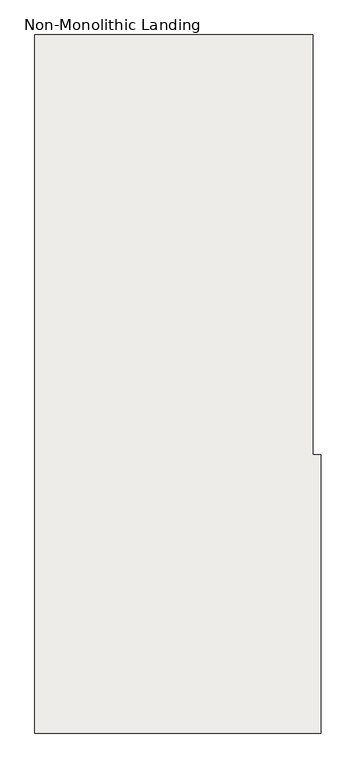
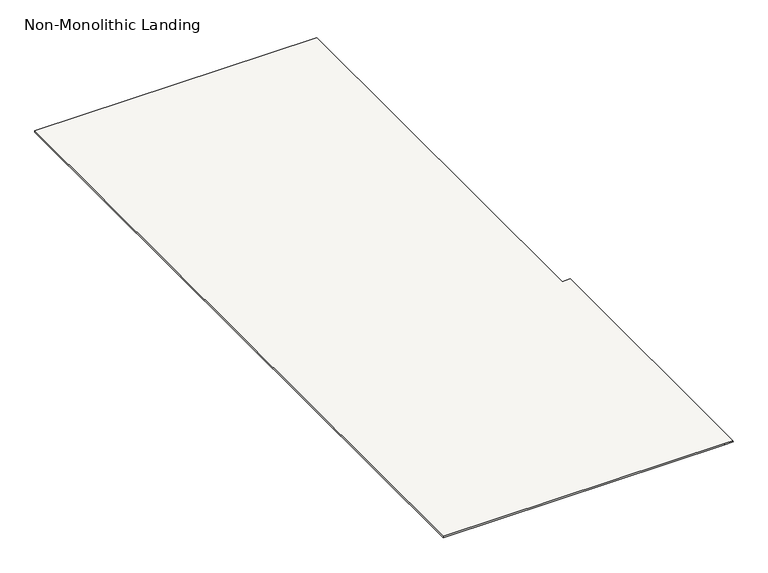
"""IFC4 building model written with IfcOpenShell, lengths in millimetres: slab geometry, Non-Monolithic Landing."""

import ifcopenshell
import ifcopenshell.guid

model = None  # the IFC model being written
_history = None  # IfcOwnerHistory: only IFC2X3 demands one
_inside = {}  # id of a spatial element -> (the spatial element, [elements in it])
_under = {}  # id of a project, library or spatial element -> (it, [spatial elements below it])
_declared = {}  # id of a project -> (the project, [libraries it declares])
_typed = {}  # id of a type object -> (the type object, [elements of that type])
_made_of = {}  # id of a material, layer set ... -> (it, [elements and type objects made of it])


def new_model(schema):
    """Start an empty IFC model of exactly this schema.

    Asked for "IFC4X3", IfcOpenShell would pick the latest addendum, in which some entities
    have other attributes; the version numbers below select the first issue.
    IFC2X3 requires an IfcOwnerHistory on every rooted entity: one is made here for all.
    """
    global model, _history
    if schema == "IFC4X3":
        model = ifcopenshell.file(schema_version=(4, 3, 0, 0))
    else:
        model = ifcopenshell.file(schema=schema)
    _inside.clear()
    _under.clear()
    _declared.clear()
    _typed.clear()
    _made_of.clear()
    _history = None
    if model.schema == "IFC2X3":
        org = make("IfcOrganization", Name="unknown")
        user = make(
            "IfcPersonAndOrganization",
            ThePerson=make("IfcPerson", FamilyName="unknown"),
            TheOrganization=org,
        )
        app = make(
            "IfcApplication",
            ApplicationDeveloper=org,
            Version="unknown",
            ApplicationFullName="unknown",
            ApplicationIdentifier="unknown",
        )
        _history = make(
            "IfcOwnerHistory",
            OwningUser=user,
            OwningApplication=app,
            ChangeAction="ADDED",
            CreationDate=0,
        )
    return model


def make(cls, **values):
    """One entity of the class cls with the attributes given. An attribute that is None is left unset."""
    return model.create_entity(
        cls, **{name: value for name, value in values.items() if value is not None}
    )


def rooted(cls, **values):
    """An entity with a GlobalId (a new one), such as an element, a storey or a relation."""
    return make(cls, GlobalId=ifcopenshell.guid.new(), OwnerHistory=_history, **values)


def si_unit(unit_type, name, prefix=None):
    """IfcSIUnit, for example si_unit("LENGTHUNIT", "METRE", prefix="MILLI")."""
    return make("IfcSIUnit", UnitType=unit_type, Prefix=prefix, Name=name)


def assignment(units):
    """IfcUnitAssignment: the units of a project."""
    return None if units is None else make("IfcUnitAssignment", Units=units)


def point(xyz):
    """IfcCartesianPoint."""
    return None if xyz is None else make("IfcCartesianPoint", Coordinates=xyz)


def direction(xyz):
    """IfcDirection."""
    return None if xyz is None else make("IfcDirection", DirectionRatios=xyz)


def frame(location, z_axis=None, x_axis=None):
    """IfcAxis2Placement3D, a coordinate frame: its origin and axes. An axis left out is left unset."""
    return make(
        "IfcAxis2Placement3D",
        Location=point(location),
        Axis=direction(z_axis),
        RefDirection=direction(x_axis),
    )


def origin():
    """The frame at (0, 0, 0) with its axes left unset."""
    return frame((0.0, 0.0, 0.0))


def place(relative_to, where):
    """IfcLocalPlacement: puts the frame where relative to a parent placement (None: the world)."""
    return make(
        "IfcLocalPlacement", PlacementRelTo=relative_to, RelativePlacement=where
    )


def context(
    kind, dimensions, precision=None, world=None, true_north=None, identifier=None
):
    """IfcGeometricRepresentationContext, for example the 3D "Model" context."""
    return make(
        "IfcGeometricRepresentationContext",
        ContextIdentifier=identifier,
        ContextType=kind,
        CoordinateSpaceDimension=dimensions,
        Precision=precision,
        WorldCoordinateSystem=world,
        TrueNorth=true_north,
    )


def project(units=None, contexts=None):
    """IfcProject with its units and contexts."""
    return rooted(
        "IfcProject",
        Name="project",
        RepresentationContexts=contexts,
        UnitsInContext=assignment(units),
    )


def spatial(cls, under=None, at=None, **own):
    """A site, building, storey or space (cls), placed at a placement, below another one or the project."""
    s = rooted(cls, ObjectPlacement=at, **own)
    if under is not None:
        _under.setdefault(under.id(), (under, []))[1].append(s)
    return s


def faces_of(points, faces, orient=None, outer=None):
    """IfcFace entities. A face is a list of loops; a loop is a list of indices into points, from 0.

    orient and outer hold one flag for each loop. By default every Orientation is true, the
    first loop of a face is its IfcFaceOuterBound and the others are IfcFaceBound.
    """
    made = []
    for i, loops in enumerate(faces):
        bounds = []
        for j, loop in enumerate(loops):
            is_outer = j == 0 if outer is None else outer[i][j]
            bounds.append(
                make(
                    "IfcFaceOuterBound" if is_outer else "IfcFaceBound",
                    Bound=make("IfcPolyLoop", Polygon=[points[k] for k in loop]),
                    Orientation=True if orient is None else orient[i][j],
                )
            )
        made.append(make("IfcFace", Bounds=bounds))
    return made


def faceted_brep(points, faces, orient=None, outer=None, voids=None):
    """IfcFacetedBrep: a solid bounded by flat faces; with voids (closed shells), ...WithVoids."""
    shared = [point(p) for p in points]
    hull = make("IfcClosedShell", CfsFaces=faces_of(shared, faces, orient, outer))
    if voids is None:
        return make("IfcFacetedBrep", Outer=hull)
    return make(
        "IfcFacetedBrepWithVoids",
        Outer=hull,
        Voids=[
            make(cls, CfsFaces=faces_of(shared, fs, o, b)) for cls, fs, o, b in voids
        ],
    )


def shape(context_of_items, identifier, shape_type, items):
    """IfcShapeRepresentation: the items that make up one representation, for example the "Body"."""
    return make(
        "IfcShapeRepresentation",
        ContextOfItems=context_of_items,
        RepresentationIdentifier=identifier,
        RepresentationType=shape_type,
        Items=items,
    )


def source(mapping_origin, context_of_items, identifier, shape_type, items):
    """IfcRepresentationMap: a shape defined once, which mapped items show again and again."""
    return make(
        "IfcRepresentationMap",
        MappingOrigin=mapping_origin,
        MappedRepresentation=shape(context_of_items, identifier, shape_type, items),
    )


def transform(
    local_origin,
    x_axis=None,
    y_axis=None,
    z_axis=None,
    scale=None,
    scale2=None,
    scale3=None,
    uniform=True,
):
    """IfcCartesianTransformationOperator3D, or its non-uniform kind. x_axis, y_axis, z_axis: its Axis1, 2, 3."""
    if uniform:
        return make(
            "IfcCartesianTransformationOperator3D",
            Axis1=direction(x_axis),
            Axis2=direction(y_axis),
            LocalOrigin=point(local_origin),
            Scale=scale,
            Axis3=direction(z_axis),
        )
    return make(
        "IfcCartesianTransformationOperator3DnonUniform",
        Axis1=direction(x_axis),
        Axis2=direction(y_axis),
        LocalOrigin=point(local_origin),
        Scale=scale,
        Axis3=direction(z_axis),
        Scale2=scale2,
        Scale3=scale3,
    )


def mapped(mapping_source, mapping_target):
    """IfcMappedItem: shows the shape of a source again, moved by a transform."""
    return make(
        "IfcMappedItem", MappingSource=mapping_source, MappingTarget=mapping_target
    )


def made_of(thing, what):
    """Note that an element or type object is made of a material, layer set ...; save() writes the relation."""
    if what is not None:
        _made_of.setdefault(what.id(), (what, []))[1].append(thing)
    return thing


def element(
    cls,
    number,
    at=None,
    inside=None,
    cuts=None,
    type_object=None,
    material=None,
    context=None,
    identifier="Body",
    shape_type=None,
    held_by="IfcProductDefinitionShape",
    body=None,
    shapes=None,
    **own,
):
    """One element of the class cls, such as IfcWall. Its Tag is "e" and its number.

    at: its placement. inside: the storey or other place that contains it. cuts: it is an
    opening in that element (IfcRelVoidsElement). A single representation is given by context,
    identifier, shape_type and body (its items); several are given by shapes. held_by: the class
    of the entity that holds the representations. save() writes the other relations.
    """
    e = rooted(cls, Tag="e%d" % number, ObjectPlacement=at, **own)
    if body is not None:
        shapes = [shape(context, identifier, shape_type, body)]
    if shapes is not None:
        e.Representation = make(held_by, Representations=shapes)
    if inside is not None:
        _inside.setdefault(inside.id(), (inside, []))[1].append(e)
    if cuts is not None:
        rooted(
            "IfcRelVoidsElement", RelatingBuildingElement=cuts, RelatedOpeningElement=e
        )
    if type_object is not None:
        _typed.setdefault(type_object.id(), (type_object, []))[1].append(e)
    return made_of(e, material)


def aggregate(whole, parts):
    """IfcRelAggregates: a whole, such as a stair, and the parts it consists of."""
    return rooted("IfcRelAggregates", RelatingObject=whole, RelatedObjects=parts)


def save(model, path):
    """Write the relations noted so far, then the file.

    IfcRelAggregates (storeys below a building ...), IfcRelContainedInSpatialStructure (elements
    in a storey), IfcRelDefinesByType, IfcRelAssociatesMaterial and IfcRelDeclares: one each for
    every whole, place, type object, material and project.
    """
    for whole, parts in _under.values():
        aggregate(whole, parts)
    for where, things in _inside.values():
        rooted(
            "IfcRelContainedInSpatialStructure",
            RelatedElements=things,
            RelatingStructure=where,
        )
    for kind, things in _typed.values():
        rooted("IfcRelDefinesByType", RelatedObjects=things, RelatingType=kind)
    for what, things in _made_of.values():
        rooted("IfcRelAssociatesMaterial", RelatedObjects=things, RelatingMaterial=what)
    for by, libraries in _declared.values():
        rooted("IfcRelDeclares", RelatingContext=by, RelatedDefinitions=libraries)
    model.write(path)


def non_monolithic_landing_917043f4(model_context):
    return source(origin(), model_context, "Body", "Brep", [
        faceted_brep([(13356.0599092, 10370.4345331, 12058.8235294), (13356.9099092, 10370.4345331, 12052.8235294), (13356.9099092, 11470.4345331, 12052.8235294), (13356.0599092, 11470.4345331, 12058.8235294), (13325.0, 13130.4345331, 12058.8235294), (12225.0, 13130.4345331, 12058.8235294), (12225.0, 10370.4345331, 12058.8235294), (13325.0, 10370.4345331, 12058.8235294), (13325.0, 11470.4345331, 12058.8235294), (13325.0, 12030.4345331, 12058.8235294), (12225.0, 10370.4345331, 12052.8235294), (12225.0, 13130.4345331, 12052.8235294), (13324.15, 13130.4345331, 12052.8235294), (13324.15, 12030.4345331, 12052.8235294), (13325.0, 12030.4345331, 12052.8235294), (13325.0, 11470.4345331, 12052.8235294), (13325.0, 10370.4345331, 12052.8235294)], [[[0, 1, 2, 3]], [[4, 5, 6, 7, 0, 3, 8, 9]], [[10, 11, 12, 13, 14, 15, 2, 1, 16]], [[9, 8, 15, 14]], [[0, 7, 16, 1]], [[7, 6, 10, 16]], [[6, 5, 11, 10]], [[5, 4, 12, 11]], [[13, 9, 14]], [[9, 13, 12, 4]], [[8, 3, 2, 15]]]),
    ])


if __name__ == "__main__":
    model = new_model("IFC4")
    model_context = context("Model", 3, world=origin())
    ifc_project = project(units=[si_unit("LENGTHUNIT", "METRE", prefix="MILLI")], contexts=[model_context])
    site = spatial("IfcSite", under=ifc_project)
    building = spatial("IfcBuilding", under=site)
    placement = place(None, origin())
    non_monolithic_landing_shape = non_monolithic_landing_917043f4(model_context)
    element("IfcSlab", 1, ObjectType="Non-Monolithic Landing", at=placement, inside=building, context=model_context, shape_type="MappedRepresentation", body=[
        mapped(non_monolithic_landing_shape, transform((0.0, 0.0, 0.0), x_axis=(1.0, 0.0, 0.0), y_axis=(0.0, 1.0, 0.0), z_axis=(0.0, 0.0, 1.0))),
    ])
    save(model, "model.ifc")

# Revit data of these elements
# Element 1 (IfcSlab, "Non-Monolithic Landing")
#   Materials on its faces: "Steel, Paint Finish, Dark Gray"
# Materials
#   "Steel, Paint Finish, Dark Gray": class "Metal", colour RGB 89 89 89, transparency 0, Description = "Steel, paint finish, dark gray, glossy", Cost = 0
